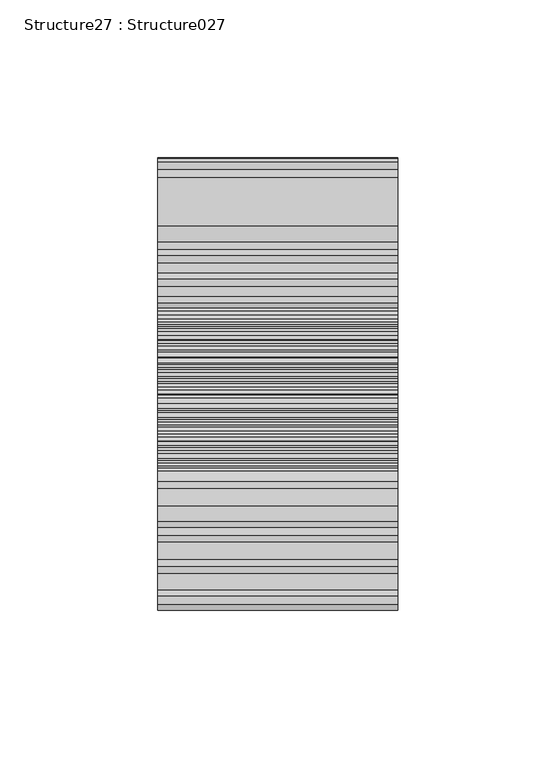
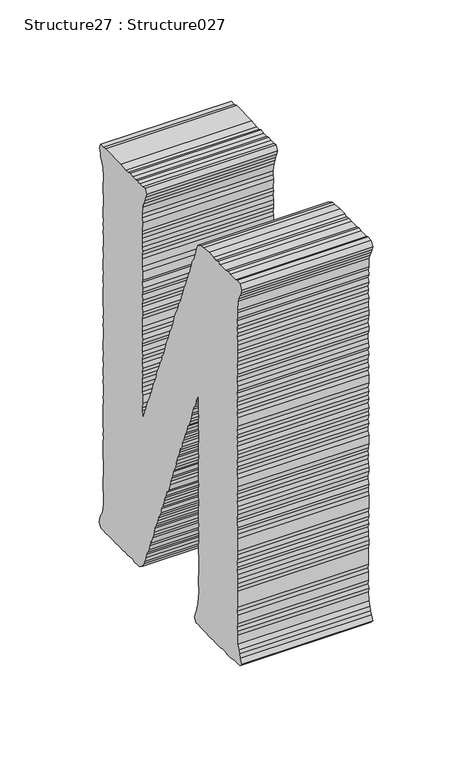
"""IFC4 building model written with IfcOpenShell, lengths in millimetres: proxy geometry, Structure27 : Structure027."""

from ifc_helpers import new_model, si_unit, frame, origin, place, context, project, spatial, polyline, outline, extrude, source, transform, mapped, element, save


def structure27_structure027_78d25ec5(model_context):
    return source(origin(), model_context, "Body", "SweptSolid", [
        extrude(outline(polyline([(4.3730473, 0.0), (7.5523619, 0.4888648), (9.447333, 0.5296799), (14.6047587, 1.6773315), (17.1469856, -0.2386542), (16.4846309, -2.6527648), (16.4531781, -5.1432884), (15.7164154, -10.3515786), (15.7605694, -12.2350435), (15.3716005, -14.9847255), (14.7622669, -17.0966038), (14.677793, -19.8893596), (14.0284831, -24.4794328), (13.106131, -26.5359087), (12.6726644, -29.6001516), (13.0313794, -31.5281142), (12.6852469, -33.9749789), (11.3723834, -38.7920416), (10.6785758, -43.6966757), (8.2899903, -45.2248832), (5.7436878, -43.3074653), (3.6878134, -42.3869096), (1.6160177, -41.4760804), (-0.9598187, -39.8642172), (-6.1210947, -38.8132496), (-8.6141347, -38.7814407), (-10.6708479, -37.8607664), (-13.170615, -37.8160273), (-18.3680005, -37.0808073), (-20.4775997, -36.4735072), (-22.9689784, -36.4299548), (-32.7673419, -35.0438823), (-35.2553488, -35.0127853), (-37.7173124, -34.6645169), (-40.117163, -34.0041795), (-42.8794274, -33.6134307), (-45.2801002, -32.9649555), (-47.8159767, -33.2359639), (-49.5807774, -32.3565834), (-52.4169547, -32.5851114), (-55.1213001, -31.8817003), (-57.3232664, -31.8910666), (-64.9775824, -30.8082901), (-67.3816272, -30.1473594), (-69.8251365, -29.8017016), (-71.7133807, -29.8554468), (-74.6886118, -28.8048393), (-76.5273254, -28.5447356), (-79.6822576, -28.7281727), (-82.125767, -28.3825148), (-84.2244779, -27.7647765), (-86.9447447, -27.0710917), (-89.4352846, -27.0276579), (-91.5364955, -26.4215444), (-93.7225404, -26.4211844), (-96.5251083, -26.3455898), (-101.4213541, -25.6529688), (-103.7917895, -24.6879155), (-106.2361377, -24.342139), (-108.7711752, -24.6132661), (-110.8270497, -23.6927104), (-113.9777879, -23.8767408), (-115.7761979, -23.3014829), (-118.2650437, -23.2702673), (-120.939974, -22.2621402), (-123.7895725, -22.4887697), (-125.5317249, -21.612593), (-128.3679021, -21.841121), (-130.4330037, -20.9192601), (-133.587936, -21.1026971), (-138.4934089, -20.4087709), (-140.535862, -19.4901138), (-143.0818044, -19.7596983), (-145.4421738, -18.7960689), (-147.5946094, -18.4915862), (-150.7361205, -18.6769219), (-153.0964899, -17.7132925), (-155.0359587, -18.0686685), (-157.4358093, -17.4083311), (-160.1409772, -16.7167821), (-162.9032416, -16.3260333), (-165.134623, -16.6401155), (-167.884305, -16.2511466), (-169.6398786, -15.3730714), (-172.4449795, -15.2851399), (-174.9464077, -15.2521444), (-177.6952508, -14.8632942), (-179.4810784, -14.2898162), (-182.5562261, -13.8548071), (-185.045072, -13.8235914), (-187.4071191, -12.8597247), (-189.9068861, -12.8149857), (-191.998031, -12.2102961), (-194.5422957, -12.480118), (-197.2138707, -11.4724655), (-199.1306912, -11.8310454), (-202.1537918, -11.0825433), (-204.0361642, -11.1371192), (-209.5901081, -10.6603375), (-211.8206507, -10.9745383), (-214.7861761, -12.1113996), (-216.7164178, -12.4680809), (-219.288555, -13.0317139), (-221.8062812, -10.8094615), (-221.7160705, -8.0063942), (-220.8382162, -6.2644793), (-220.099911, -1.0452842), (-220.4156708, 1.1863344), (-219.4934375, 3.2419716), (-218.7138385, 8.7530791), (-219.0297169, 10.9838591), (-218.0645286, 13.3431524), (-218.4232435, 15.2711149), (-217.7293172, 20.1765878), (-216.3307809, 25.5992852), (-216.0274849, 27.7433325), (-213.7116295, 30.8501704), (-211.7528114, 31.5116863), (-208.5894908, 31.6939367), (-206.3303556, 32.3009912), (-204.0578154, 32.918128), (-202.1266161, 33.2755295), (-199.4656022, 34.4674455), (-196.5748285, 34.9851487), (-194.3006107, 35.6020482), (-192.0556894, 35.9150707), (-189.1338392, 36.7492333), (-187.2623553, 36.7933709), (-184.6307401, 37.6685901), (-182.0527475, 38.2433734), (-179.4782287, 38.8177924), (-177.4623143, 39.7801083), (-175.2317716, 40.0943092), (-172.6438317, 40.6668298), (-170.6865562, 41.3174408), (-167.8352801, 41.5438329), (-165.4754058, 42.778348), (-163.2465244, 43.0808053), (-160.4010014, 43.3088668), (-157.7366158, 44.4883273), (-153.493514, 45.7653188), (-151.2149833, 46.3824638), (-148.7294764, 46.3397419), (-146.1070883, 47.2162663), (-143.2196863, 47.7464251), (-140.9025135, 48.6669808), (-139.2776056, 49.0668545), (-136.0940968, 49.5551261), (-134.4691726, 49.9430188), (-131.8468009, 50.8315242), (-128.9601027, 51.3506595), (-126.7295601, 51.6648603), (-124.4553423, 52.2817598), (-121.6166322, 52.497951), (-119.8605963, 53.8187403), (-117.3742504, 53.7758999), (-115.0151987, 54.9985527), (-112.1656002, 55.2251821), (-109.5338662, 56.1012402), (-107.2697144, 56.7195636), (-104.9954966, 57.3364631), (-103.1139466, 57.3791767), (-99.8767132, 58.180704), (-97.561218, 59.101497), (-95.2870001, 59.7183965), (-92.7393637, 59.9757628), (-90.2076815, 60.2473646), (-88.2479059, 60.9096006), (-85.662466, 61.4704962), (-83.0409168, 62.3471392), (-81.0275351, 63.3217921), (-76.2492374, 63.894198), (-73.9892798, 64.5131149), (-70.7528688, 65.3027798), (-68.4659498, 65.9187383), (-68.9984941, 66.6118257), (-71.3689294, 67.576879), (-73.1984158, 67.8356774), (-76.3483152, 67.6515284), (-81.254627, 68.3455733), (-83.0060063, 69.2230552), (-85.7590437, 69.6124987), (-88.2453894, 69.6553393), (-91.016881, 70.0473933), (-93.5099209, 70.0792023), (-95.2520732, 70.9553789), (-97.7971768, 70.6856758), (-100.158385, 71.6494237), (-102.6161545, 71.9970988), (-105.4514929, 71.7684522), (-107.5510425, 72.3863092), (-110.5707714, 73.1223557), (-112.4573543, 73.0803541), (-114.9361341, 73.1101458), (-117.6211305, 74.1196967), (-120.1116704, 74.1631305), (-122.5131821, 74.8117243), (-127.4186551, 75.5056506), (-129.9629197, 75.2358288), (-131.7924061, 75.4946272), (-134.7584102, 76.5439294), (-136.610545, 76.8059316), (-139.1472602, 76.5350419), (-142.1653278, 77.282832), (-144.048539, 77.2283748), (-146.48366, 77.5728461), (-149.4714737, 78.6252334), (-151.389133, 78.2667723), (-156.2954448, 78.9608172), (-159.3135124, 79.7086073), (-164.2189852, 80.4025335), (-166.3067749, 81.0067483), (-168.8560726, 80.7376385), (-170.9547834, 81.3553768), (-173.7036266, 81.7442271), (-176.4322817, 82.4390984), (-178.9236605, 82.4826509), (-180.7195375, 83.0455719), (-186.3037191, 83.2057756), (-188.6791875, 84.1715408), (-191.121858, 84.51708), (-195.8538452, 84.2478555), (-198.7371717, 83.7162647), (-200.976119, 83.4152314), (-203.8971303, 82.58095), (-206.4750042, 82.0070056), (-209.023103, 83.923822), (-208.4144731, 86.0246769), (-207.9811252, 89.088081), (-207.9386653, 91.5898817), (-207.0742322, 93.3336952), (-206.6408843, 96.3970993), (-206.9003865, 98.9296369), (-206.0344108, 100.6843552), (-205.6866171, 103.1429634), (-205.6001054, 108.1215268), (-203.4345525, 123.430159), (-202.4811241, 125.8030944), (-202.4352924, 128.2924395), (-199.8465137, 128.8648413), (-196.9149577, 127.5115352), (-195.1150051, 126.947182), (-192.5383301, 125.3352002), (-190.220797, 124.0687535), (-185.1015186, 122.7148499), (-183.2636439, 122.4548649), (-180.1087115, 122.6383019), (-175.520316, 121.9892294), (-173.1507195, 121.0242947), (-167.953334, 120.2890746), (-166.0659288, 120.3429385), (-160.8467337, 119.6046333), (-158.4561103, 118.9456012), (-155.9672644, 118.9143855), (-153.8551324, 118.2947487), (-151.3662865, 118.2635331), (-148.6485197, 117.5582234), (-143.7564681, 116.8661957), (-141.2063316, 117.1351869), (-136.401614, 115.825781), (-133.8573493, 116.0956029), (-131.1505038, 115.4038166), (-128.9947128, 115.0988593), (-126.2895285, 114.3953295), (-124.372708, 114.7539093), (-121.2958827, 114.3186629), (-119.2408471, 113.3982258), (-116.7520012, 113.3670102), (-111.5411945, 112.6298916), (-109.3459224, 112.6282263), (-106.6399157, 111.9365587), (-104.8549269, 111.3631994), (-102.3979964, 111.015643), (-99.5996226, 110.9406416), (-97.5000729, 110.3227847), (-94.6983438, 110.2473087), (-91.9797382, 109.5418804), (-87.0885254, 108.8499714), (-84.8571439, 109.1640536), (-79.951671, 108.4701274), (-77.8815365, 107.5475544), (-74.7878948, 107.4307846), (-72.915572, 107.4748036), (-70.5451366, 106.5097503), (-68.0529356, 106.47806), (-65.6043932, 106.1316902), (-62.5770984, 105.3825948), (-60.7031144, 105.4383573), (-57.6800139, 104.6898552), (-52.7787351, 103.9965223), (-50.5473536, 104.3106045), (-48.4914792, 103.3900488), (-45.3793833, 103.2706684), (-42.8796162, 103.2259294), (-40.7926655, 102.6218332), (-33.1375106, 101.5389381), (-31.0253784, 100.9193012), (-28.2320376, 100.8450118), (-26.4327887, 100.2696353), (-23.3257258, 100.1509669), (-21.4534031, 100.1949859), (-18.4336742, 99.4589393), (-16.2333691, 99.456562), (-13.7898599, 99.1109042), (-11.7339854, 98.1903485), (-4.0788305, 97.1074534), (-1.2720684, 97.0312655), (0.9005553, 97.032804), (3.6342434, 96.3372206), (5.5065661, 96.3812396), (8.1764636, 95.3738244), (13.3872703, 94.6367058), (17.7618602, 94.6476106), (20.9411747, 95.1364755), (22.9663164, 96.0974861), (26.1507825, 96.5864779), (28.079363, 96.9314156), (30.5786349, 94.7117737), (30.2754575, 92.5685652), (30.2749952, 90.3697005), (29.5386948, 87.3602749), (29.2355174, 85.2170665), (28.5303263, 82.5001385), (28.8890413, 80.5721759), (28.1510797, 77.5510067), (27.8922813, 75.7215204), (27.7634284, 72.6150425), (26.8410764, 70.5585666), (27.1139998, 68.0241306), (26.1044324, 65.3511152), (25.8439727, 63.5098852), (26.1170149, 60.9762879), (25.4218897, 58.2579361), (25.1185936, 56.1138887), (22.5319713, 53.3550859), (20.2677008, 52.7359237), (17.608348, 51.5557514), (15.408043, 51.5581286), (12.5290294, 51.0267833), (10.1984352, 50.1081262), (7.8956411, 49.1863921), (5.0460426, 48.9597626), (2.4152662, 48.0844248), (-2.1316104, 46.8495496), (-4.3966012, 46.2313449), (-6.2915723, 46.1905297), (-9.4708868, 45.7016648), (-11.4440837, 45.0413274), (-14.1042751, 43.8612736), (-16.2919813, 43.8498902), (-18.9269518, 42.9751456), (-21.2004495, 42.3572886), (-23.5032437, 41.4355545), (-26.3175716, 41.5247913), (-28.3217262, 40.5488332), (-30.9526212, 39.6726565), (-33.1302779, 39.67183), (-35.7509882, 38.7950682), (-37.6770358, 38.4377936), (-40.254206, 37.8748726), (-42.6241463, 36.6417814), (-47.4762381, 35.4509375), (-49.9634227, 35.4938966), (-52.5850905, 34.6164147), (-54.5673958, 33.9582214), (-57.7080681, 33.7727671), (-59.3766512, 33.0701948), (-61.9932862, 32.1920009), (-64.5854203, 31.6200737), (-66.772304, 31.6205524), (-69.6513177, 31.0892071), (-71.6186591, 30.4400199), (-74.2410307, 29.5515146), (-76.1670784, 29.19424), (-79.146025, 28.0592772), (-81.6365648, 28.102711), (-84.2674598, 27.2265343), (-86.4845812, 26.9104349), (-89.1153575, 26.0350971), (-90.7318771, 25.6340368), (-93.967568, 24.8434143), (-96.1964493, 24.540957), (-98.2434403, 23.2621816), (-100.5295368, 22.6580854), (-103.1032167, 22.0835477), (-105.6483202, 21.8138445), (-107.5634794, 21.4670083), (-110.4433155, 20.9238006), (-113.1220798, 19.7455186), (-115.3534613, 19.4314364), (-117.3206841, 18.7830881), (-119.898558, 18.2091437), (-122.529453, 17.332967), (-120.1161813, 16.670731), (-117.9368634, 16.6833012), (-114.8617157, 16.248292), (-112.762166, 15.630435), (-110.3606543, 14.9818412), (-108.1746094, 14.981481), (-103.2682976, 14.2874362), (-100.2485687, 13.5513896), (-95.9613129, 12.9449161), (-92.8517171, 12.8139109), (-90.977733, 12.8696734), (-88.5644613, 12.2074374), (-85.8584545, 11.5157699), (-83.3225781, 11.7867783), (-78.1168044, 11.0503717), (-75.7035326, 10.3881356), (-73.5158264, 10.3995192), (-70.8114809, 9.696108), (-68.6968487, 9.088096), (-66.1660053, 9.3598164), (-63.4121292, 8.9702542), (-61.3041912, 8.3512106), (-59.2130462, 7.7465211), (-56.7552768, 7.3988461), (-54.5692319, 7.398486), (-51.5058278, 6.965138), (-49.0136266, 6.9334479), (-46.6137761, 6.2731104), (-44.4999827, 5.6652171), (-41.9641064, 5.9362256), (-39.3025973, 4.9299971), (-34.4013185, 4.2366641), (-32.2144347, 4.2361854), (-27.3089619, 3.5422591), (-25.2085897, 2.9362644), (-14.7911704, 1.4626205), (-12.6185467, 1.4641589), (-9.7975245, 1.3859539), (-7.6677374, 1.084675), (-5.5984416, 0.1622208), (-3.1540935, -0.1835557), (0.0, 0.0), (4.3730473, 0.0)])), frame((-35624.0862846, 276095.3076568, 3999.8318725), z_axis=(1.0, 0.0, 1.354250045437766e-12), x_axis=(1.3435374844757662e-12, 0.14006512962532752, -0.9901422925332704)), (0.0, 0.0, 1.0), 76.2),
    ])


if __name__ == "__main__":
    model = new_model("IFC4")
    model_context = context("Model", 3, world=origin())
    ifc_project = project(units=[si_unit("LENGTHUNIT", "METRE", prefix="MILLI")], contexts=[model_context])
    site = spatial("IfcSite", under=ifc_project)
    building = spatial("IfcBuilding", under=site)
    placement = place(None, origin())
    structure27_structure027_shape = structure27_structure027_78d25ec5(model_context)
    element("IfcBuildingElementProxy", 1, Name="Structure27 : Structure027", ObjectType="Structure27 : Structure027", at=placement, inside=building, context=model_context, shape_type="MappedRepresentation", body=[
        mapped(structure27_structure027_shape, transform((0.0, 0.0, 0.0), x_axis=(1.0, 0.0, 0.0), y_axis=(0.0, 1.0, 0.0), z_axis=(0.0, 0.0, 1.0))),
    ])
    save(model, "model.ifc")

# Revit data of these elements
# Type "Structure27 : Structure027"
#   NameOverride = "Structure027"
# Element 1 (IfcBuildingElementProxy, "Structure27 : Structure027")
#   Materials on its faces: "BRUSHED ALUMINUM LETTERING"
# Materials
#   "BRUSHED ALUMINUM LETTERING": class "Unassigned", colour RGB 169 181 186, transparency 0, Cost = 0
